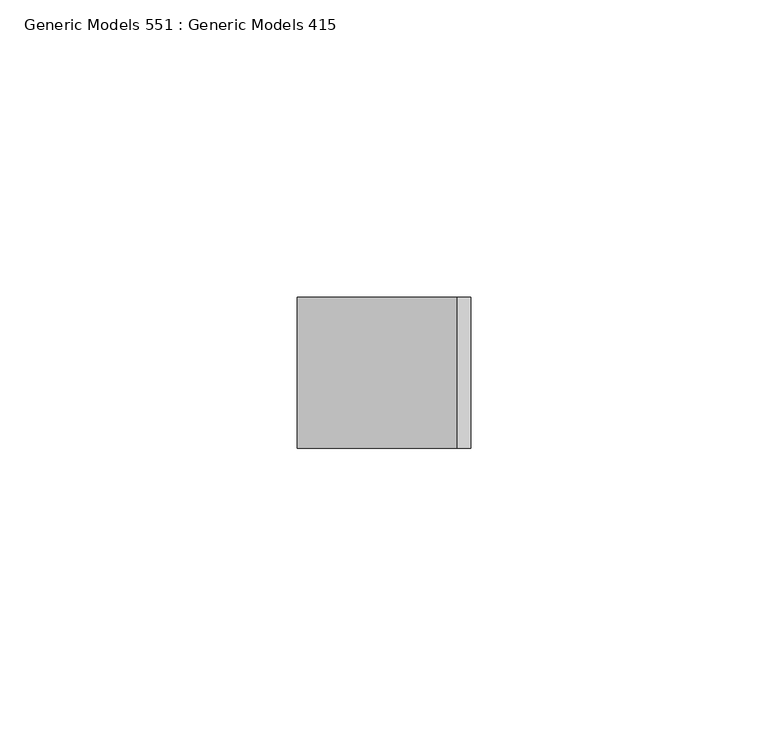
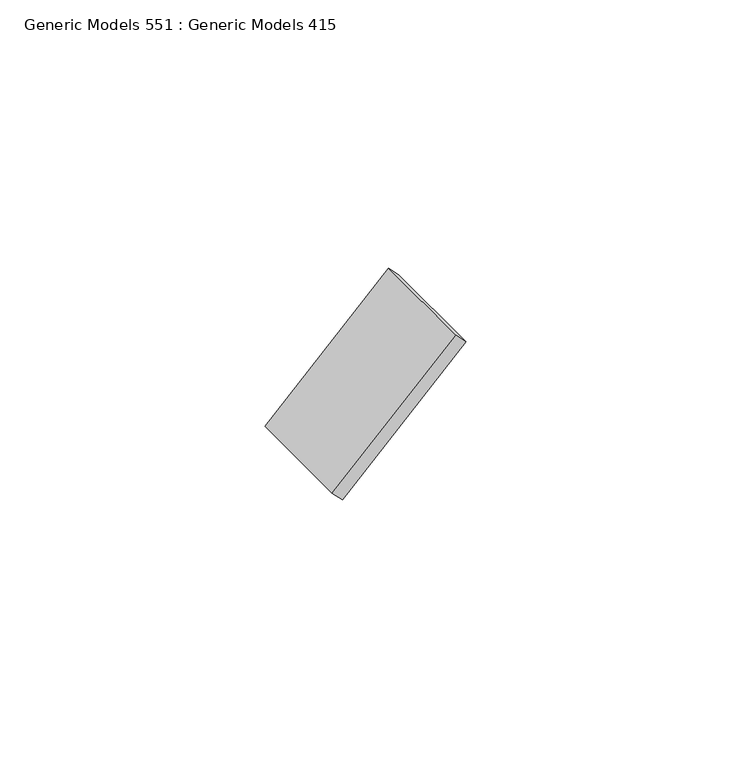
"""IFC4 building model written with IfcOpenShell, lengths in millimetres: proxy geometry, Generic Models 551 : Generic Models 415."""

from ifc_helpers import new_model, si_unit, frame, origin, place, context, project, spatial, polyline, outline, extrude, source, transform, mapped, element, save


def generic_models_551_generic_models_415_548926b9(model_context):
    return source(origin(), model_context, "Body", "SweptSolid", [
        extrude(outline(polyline([(0.0, -3.175), (0.0, 0.0), (25.4, 0.0), (25.4, -3.175), (0.0, -3.175)])), frame((7848.0411784, 4501.3863946, 124686.3849742), z_axis=(0.7071067811867181, 0.0, 0.707106781186377), x_axis=(0.0, -1.0, 0.0)), (0.0, 0.0, 1.0), 38.1),
    ])


if __name__ == "__main__":
    model = new_model("IFC4")
    model_context = context("Model", 3, world=origin())
    ifc_project = project(units=[si_unit("LENGTHUNIT", "METRE", prefix="MILLI")], contexts=[model_context])
    site = spatial("IfcSite", under=ifc_project)
    building = spatial("IfcBuilding", under=site)
    placement = place(None, origin())
    generic_models_551_generic_models_415_shape = generic_models_551_generic_models_415_548926b9(model_context)
    element("IfcBuildingElementProxy", 1, Name="Generic Models 551 : Generic Models 415", ObjectType="Generic Models 551 : Generic Models 415", at=placement, inside=building, context=model_context, shape_type="MappedRepresentation", body=[
        mapped(generic_models_551_generic_models_415_shape, transform((0.0, 0.0, 0.0), x_axis=(1.0, 0.0, 0.0), y_axis=(0.0, 1.0, 0.0), z_axis=(0.0, 0.0, 1.0))),
    ])
    save(model, "model.ifc")

# Revit data of these elements
# Element 1 (IfcBuildingElementProxy, "Generic Models 551 : Generic Models 415")
#   Materials on its faces: "_WELDED STEEL TABS FOR LOUVER ATTACHMENT"
# Materials
#   "_WELDED STEEL TABS FOR LOUVER ATTACHMENT": class "Metal", colour RGB 199 199 199, transparency 0, Description = "Structural steel 50ksi", Cost = 0
